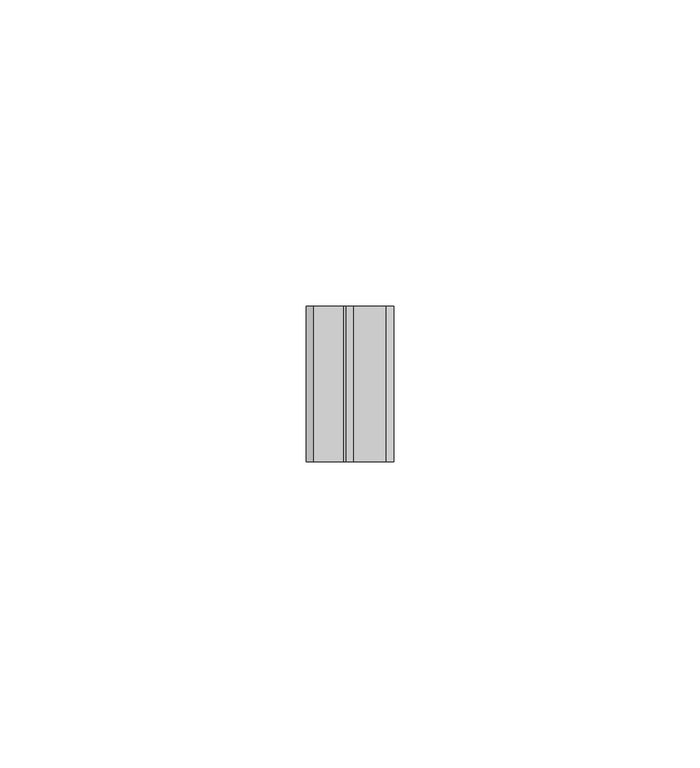
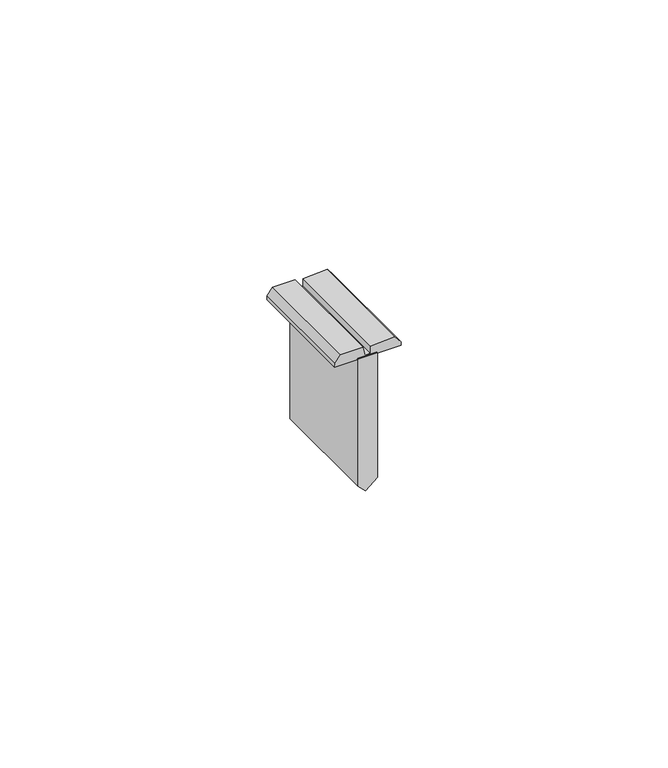
"""IFC4 building model written with IfcOpenShell, lengths in millimetres: proxy geometry, FASTENER005 5969 : FASTENER005 5969."""

from ifc_helpers import new_model, si_unit, frame, origin, place, context, project, spatial, polyline, outline, extrude, source, transform, mapped, element, save


def generic_models_4a0cef2c(model_context):
    return source(origin(), model_context, "Body", "SweptSolid", [
        extrude(outline(polyline([(42579.6987049, 5977.3107075), (42550.7399648, 5977.3107075), (42549.1244121, 5978.9677221), (42551.3049701, 5981.517626), (42579.6987049, 5981.517626), (42579.6987049, 5977.3107075)])), frame((0.0, -1078.2906574, 0.0), z_axis=(0.0, 1.0, 0.0), x_axis=(0.0, 0.0, 1.0)), (0.0, 0.0, 1.0), 25.4),
        extrude(outline(polyline([(42579.6987049, 5986.5634932), (42580.508527, 5986.5634932), (42582.1023984, 5985.3247911), (42581.7061629, 5980.0391089), (42580.1167322, 5980.0391089), (42580.1167322, 5978.792004), (42582.1288635, 5978.3957685), (42582.1288635, 5973.5166866), (42580.5349921, 5972.2779845), (42579.6987049, 5972.2671879), (42579.6987049, 5986.5634932)])), frame((0.0, -1078.2906574, 0.0), z_axis=(0.0, 1.0, 0.0), x_axis=(0.0, 0.0, 1.0)), (0.0, 0.0, 1.0), 25.4),
    ])


if __name__ == "__main__":
    model = new_model("IFC4")
    model_context = context("Model", 3, world=origin())
    ifc_project = project(units=[si_unit("LENGTHUNIT", "METRE", prefix="MILLI")], contexts=[model_context])
    site = spatial("IfcSite", under=ifc_project)
    building = spatial("IfcBuilding", under=site)
    placement = place(None, origin())
    generic_models_shape = generic_models_4a0cef2c(model_context)
    element("IfcBuildingElementProxy", 1, Name="FASTENER005 5969 : FASTENER005 5969", ObjectType="FASTENER005 5969 : FASTENER005 5969", at=placement, inside=building, context=model_context, shape_type="MappedRepresentation", body=[
        mapped(generic_models_shape, transform((0.0, 0.0, 0.0), x_axis=(1.0, 0.0, 0.0), y_axis=(0.0, 1.0, 0.0), z_axis=(0.0, 0.0, 1.0))),
    ])
    save(model, "model.ifc")

# Revit data of these elements
# Type "FASTENER005 5969 : FASTENER005 5969"
#   NameOverride = "FASTENER005"
# Element 1 (IfcBuildingElementProxy, "FASTENER005 5969 : FASTENER005 5969")
#   Materials on its faces: "ENGINEERED PANCAKE HEAD FASTENER (NOT BY AEP-SPAN) @ 12\" O.C."
# Materials
#   "ENGINEERED PANCAKE HEAD FASTENER (NOT BY AEP-SPAN) @ 12\" O.C.": class "Unassigned", colour RGB 255 255 255, transparency 0
